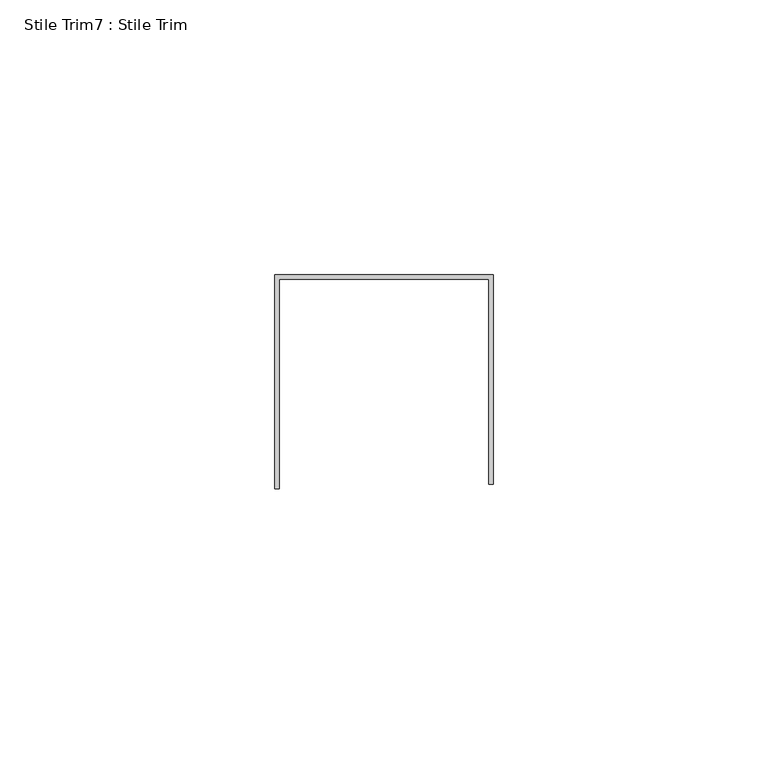
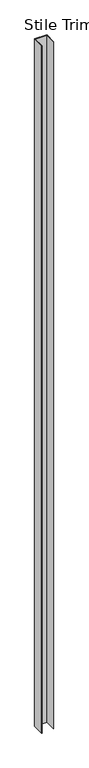
"""IFC4 building model written with IfcOpenShell, lengths in millimetres: proxy geometry, Stile Trim7 : Stile Trim."""

from ifc_helpers import new_model, si_unit, frame, origin, place, context, project, spatial, polyline, outline, extrude, source, transform, mapped, element, save


def stile_trim7_stile_trim_ecce4863(model_context):
    return source(origin(), model_context, "Body", "SweptSolid", [
        extrude(outline(polyline([(587327.0060739, -534108.5789841), (587366.6808739, -534108.5789841), (587366.6808739, -534146.6789841), (587365.8934739, -534146.6789841), (587365.8934739, -534109.3663841), (587327.7934739, -534109.3663841), (587327.7934739, -534147.4663841), (587327.0060739, -534147.4663841), (587327.0060739, -534108.5789841)])), frame((0.0, 0.0, 50.8), z_axis=(0.0, 0.0, 1.0), x_axis=(1.0, 0.0, 0.0)), (0.0, 0.0, 1.0), 2350.3929688),
    ])


if __name__ == "__main__":
    model = new_model("IFC4")
    model_context = context("Model", 3, world=origin())
    ifc_project = project(units=[si_unit("LENGTHUNIT", "METRE", prefix="MILLI")], contexts=[model_context])
    site = spatial("IfcSite", under=ifc_project)
    building = spatial("IfcBuilding", under=site)
    placement = place(None, origin())
    stile_trim7_stile_trim_shape = stile_trim7_stile_trim_ecce4863(model_context)
    element("IfcBuildingElementProxy", 1, Name="Stile Trim7 : Stile Trim", ObjectType="Stile Trim7 : Stile Trim", at=placement, inside=building, context=model_context, shape_type="MappedRepresentation", body=[
        mapped(stile_trim7_stile_trim_shape, transform((0.0, 0.0, 0.0), x_axis=(1.0, 0.0, 0.0), y_axis=(0.0, 1.0, 0.0), z_axis=(0.0, 0.0, 1.0))),
    ])
    save(model, "model.ifc")

# Revit data of these elements
# Element 1 (IfcBuildingElementProxy, "Stile Trim7 : Stile Trim")
#   Materials on its faces: "EDGE TRIM BY MTL PANEL MFR."
# Materials
#   "EDGE TRIM BY MTL PANEL MFR.": class "Generic", colour RGB 239 242 240, transparency 0, Cost = 0
